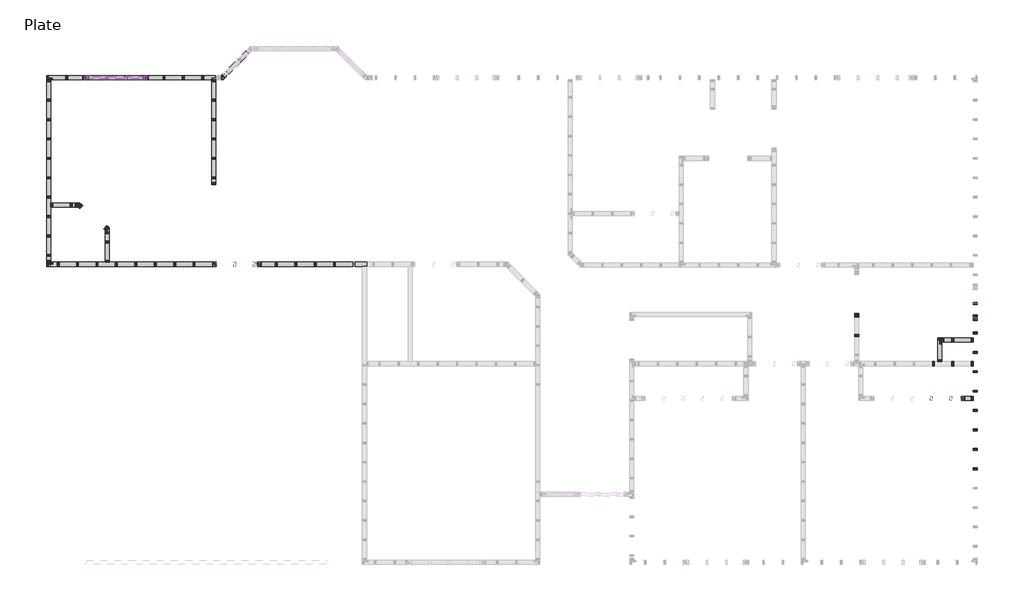
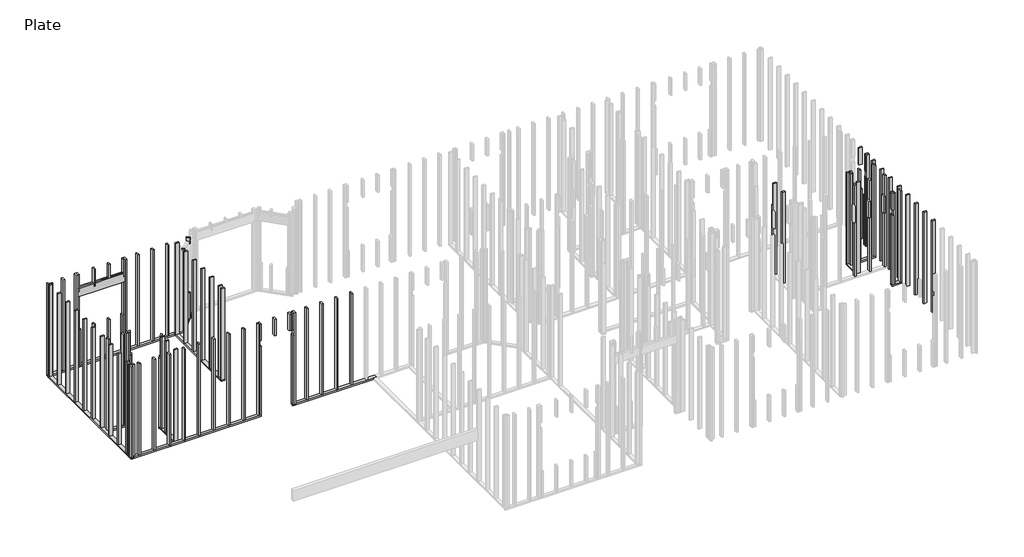
# One storey, part 3 of 5: 104 columns, 15 beams.
# Revit data of these elements (continued)
# Type "Dimension Lumber : 2x10 Header Exterior"
#   Assembly Code = "B10"
#   A = 0.0963889 SF
#   Length [instance default] = 5' - 0"
#   b = 0' - 1 1/2"
#   d = 0' - 9 1/4"
#   Structural Material [instance default] = Softwood, Lumber
# Type "Dimension Lumber : Supporting Bottom Plate"
#   Assembly Code = "B10"
#   A = 0.0364583 SF
#   Length [instance default] = 5' - 0"
#   b = 0' - 3 1/2"
#   d = 0' - 1 1/2"
#   Structural Material [instance default] = Softwood, Lumber
# Type "Dimension Lumber-Column : 2x4"
#   Int Type = "Interior"
#   Assembly Code = "B10"
#   Cost = 8.05
#   A = 0.0364583 SF
#   b = 0' - 1 1/2"
#   d = 0' - 3 1/2"
#   Structural Material [instance default] = Softwood, Lumber
# Elements 1, 2 (IfcBeam, "Dimension Lumber : 2x10 Header Exterior")
#   Comments = ""
#   Structural Material = Douglas Fir #2
#   Phase Created = New Construction
#   Materials on its faces: "Douglas Fir #2"
# Elements 3, 4, 5, 6, 7, 8, 9, 10, 11, 12, 13, 14, 15 (IfcBeam, "Dimension Lumber : Supporting Bottom Plate")
#   Structural Material = Douglas Fir #2
#   Phase Created = New Construction
#   Materials on its faces: "Douglas Fir #2"
# Elements 16, 17, 18, 19, 20, 21, 22, 23, 24, 28, 50, 52, 56, 57, 67, 68, 69, 70, 71, 72, 73, 74, 75, 76, 77, 78, 79, 80, 84, 85, 86, 87, 88, 89, 90, 91, 92, 99, 100, 101, 102, 110, 111, 112, 118, 119 (IfcColumn, "Dimension Lumber-Column : 2x4")
#   Function = "Exterior"
#   Structural Material = Douglas Fir #2
#   Phase Created = New Construction
#   Materials on its faces: "Douglas Fir #2"
# Elements 25, 26, 27, 29, 30, 31, 32, 33, 34, 35, 36, 37, 38, 39, 40, 41, 42, 43, 44, 45, 46, 47, 48, 49, 51, 53, 54, 55, 58, 59, 60, 61, 62, 63, 64, 65, 66, 81, 82, 83, 93, 94, 95, 96, 97, 98, 103, 104, 105, 106, 107, 108, 109 (IfcColumn, "Dimension Lumber-Column : 2x4")
#   Function = "Interior"
#   Structural Material = Douglas Fir #2
#   Phase Created = New Construction
#   Materials on its faces: "Douglas Fir #2"
# Elements 113, 114, 115, 116, 117 (IfcColumn, "Dimension Lumber-Column : 2x4")
#   Structural Material = Douglas Fir #2
#   Phase Created = New Construction
#   Materials on its faces: "Douglas Fir #2"
# Materials
#   "Softwood, Lumber": class "Wood", colour RGB 223 192 134, transparency 0, Description = "Pinus Echinata", Cost = 0
#   "Douglas Fir #2": class "Wood", colour RGB 223 192 134, transparency 0, Description = "Pinus Echinata", Cost = 0
